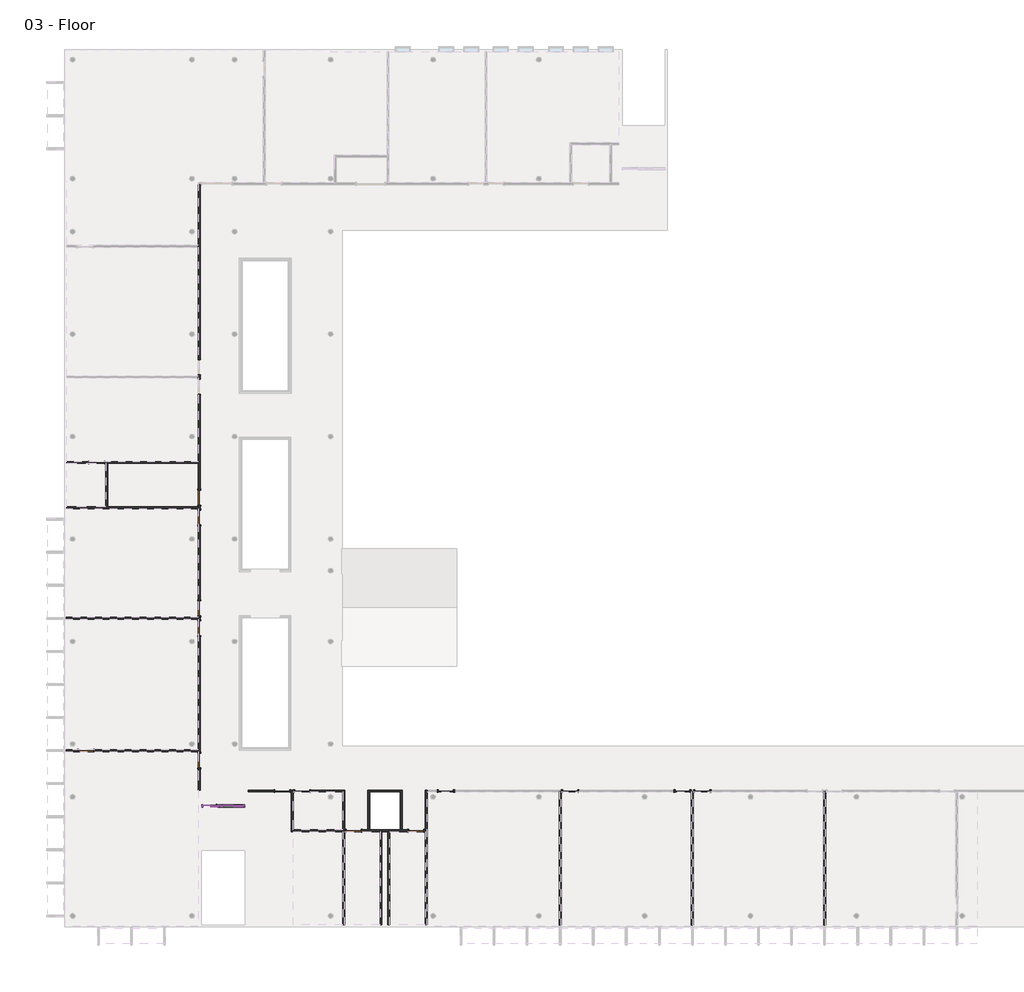
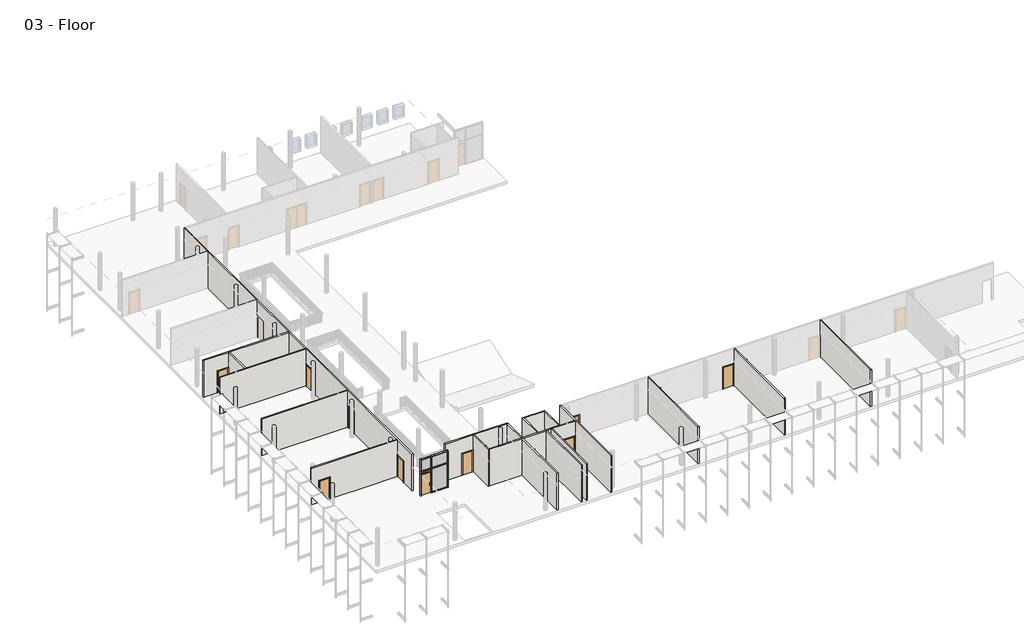
# One storey, part 1 of 4: 19 walls, 18 members, 16 doors, 4 plates.
# Revit data of these elements (continued)
# Area at (16274.088, 3147.372) mm, upper offset 0' - 0", lower offset 0' - 0"
#   Number = "24"
#   Name = "Service"
# Area at (44852.99, 3206.11) mm, upper offset 0' - 0", lower offset 0' - 0"
#   Number = "25"
#   Name = "Instruction"
# Area at (14053.66, 31558.244) mm, upper offset 0' - 0", lower offset 0' - 0"
#   Number = "27"
#   Name = "Cirrculation"
# Room at (15121.963, 31385.693) mm, phase "New Construction", upper level "03 - Floor", upper offset 8' - 0", lower offset 0' - 0"
#   Number = "318"
#   Name = "Lobby"
# Room at (27186.017, 44119.972) mm, phase "New Construction", upper level "03 - Floor", upper offset 8' - 0", lower offset 0' - 0"
#   Number = "328"
#   Name = "Corridor"
# Room at (35982.723, 48308.88) mm, phase "New Construction", upper level "03 - Floor", upper offset 8' - 0", lower offset 0' - 0"
#   Number = "327"
#   Name = "Stair"
# Room at (32631.597, 46884.651) mm, phase "New Construction", upper level "03 - Floor", upper offset 8' - 0", lower offset 0' - 0"
#   Number = "326"
#   Name = "Toilet"
# Room at (30956.034, 50151.999) mm, phase "New Construction", upper level "03 - Floor", upper offset 8' - 0", lower offset 0' - 0"
#   Number = "325"
#   Name = "Conference"
# Room at (23416.001, 49816.886) mm, phase "New Construction", upper level "03 - Floor", upper offset 8' - 0", lower offset 0' - 0"
#   Number = "324"
#   Name = "Advisors"
# Room at (18556.868, 46291.854) mm, phase "New Construction", upper level "03 - Floor", upper offset 8' - 0", lower offset 0' - 0"
#   Number = "323"
#   Name = "Electrical"
# Room at (17467.752, 49565.552) mm, phase "New Construction", upper level "03 - Floor", upper offset 8' - 0", lower offset 0' - 0"
#   Number = "322"
#   Name = "Administration"
# Room at (7330.595, 49230.439) mm, phase "New Construction", upper level "03 - Floor", upper offset 8' - 0", lower offset 0' - 0"
#   Number = "321"
#   Name = "Open Office"
# Room at (4392.01, 37166.385) mm, phase "New Construction", upper level "03 - Floor", upper offset 8' - 0", lower offset 0' - 0"
#   Number = "320"
#   Name = "Media Review"
# Room at (4643.344, 31050.58) mm, phase "New Construction", upper level "03 - Floor", upper offset 8' - 0", lower offset 0' - 0"
#   Number = "319"
#   Name = "Media Review"
# Room at (1885.015, 26610.338) mm, phase "New Construction", upper level "03 - Floor", upper offset 8' - 0", lower offset 0' - 0"
#   Number = "316"
#   Name = "Storage"
# Room at (4482.138, 26694.116) mm, phase "New Construction", upper level "03 - Floor", upper offset 8' - 0", lower offset 0' - 0"
#   Number = "317"
#   Name = "Electrical"
# Room at (4643.344, 22253.874) mm, phase "New Construction", upper level "03 - Floor", upper offset 8' - 0", lower offset 0' - 0"
#   Number = "315"
#   Name = "Instruction"
# Room at (4475.788, 14462.506) mm, phase "New Construction", upper level "03 - Floor", upper offset 8' - 0", lower offset 0' - 0"
#   Number = "314"
#   Name = "Instruction"
# Room at (4230.804, 5079.353) mm, phase "New Construction", upper level "03 - Floor", upper offset 8' - 0", lower offset 0' - 0"
#   Number = "313"
#   Name = "Instruction"
# Room at (10095.274, 5917.135) mm, phase "New Construction", upper level "03 - Floor", upper offset 8' - 0", lower offset 0' - 0"
#   Number = "312"
#   Name = "Stair"
# Room at (15540.854, 7096.379) mm, phase "New Construction", upper level "03 - Floor", upper offset 8' - 0", lower offset 0' - 0"
#   Number = "310"
#   Name = "Electrical"
# Room at (15289.52, 2566.009) mm, phase "New Construction", upper level "03 - Floor", upper offset 8' - 0", lower offset 0' - 0"
#   Number = "309"
#   Name = "Lounge"
# Room at (18221.755, 3068.677) mm, phase "New Construction", upper level "03 - Floor", upper offset 8' - 0", lower offset 0' - 0"
#   Number = "308"
#   Name = "Women"
# Room at (21489.103, 1560.671) mm, phase "New Construction", upper level "03 - Floor", upper offset 8' - 0", lower offset 0' - 0"
#   Number = "307"
#   Name = "Men"
# Room at (26013.123, 9525.945) mm, phase "New Construction", upper level "03 - Floor", upper offset 8' - 0", lower offset 0' - 0"
#   Number = "329"
#   Name = "Corridor"
# Room at (27353.574, 2901.121) mm, phase "New Construction", upper level "03 - Floor", upper offset 8' - 0", lower offset 0' - 0"
#   Number = "306"
#   Name = "Instruction"
# Room at (35480.054, 4750.59) mm, phase "New Construction", upper level "03 - Floor", upper offset 8' - 0", lower offset 0' - 0"
#   Number = "305"
#   Name = "Instruction"
# Room at (43606.535, 3236.234) mm, phase "New Construction", upper level "03 - Floor", upper offset 8' - 0", lower offset 0' - 0"
#   Number = "304"
#   Name = "Instruction"
# Room at (51314.125, 3822.681) mm, phase "New Construction", upper level "03 - Floor", upper offset 8' - 0", lower offset 0' - 0"
#   Number = "303"
#   Name = "Instruction"
# Room at (58854.159, 3655.125) mm, phase "New Construction", upper level "03 - Floor", upper offset 8' - 0", lower offset 0' - 0"
#   Number = "302"
#   Name = "Instruction"
# Room at (64886.186, 5498.244) mm, phase "New Construction", upper level "03 - Floor", upper offset 8' - 0", lower offset 0' - 0"
#   Number = "301"
#   Name = "Stair"
